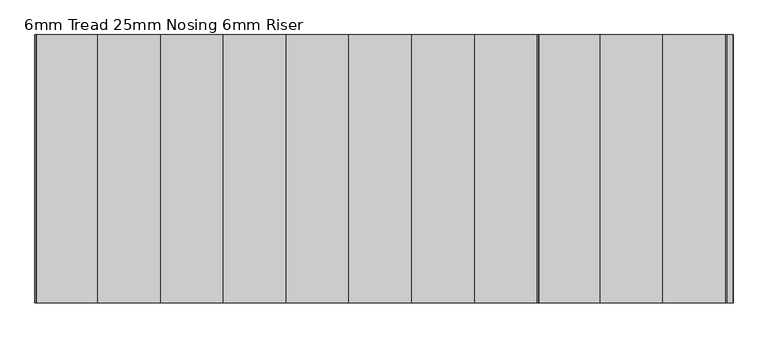
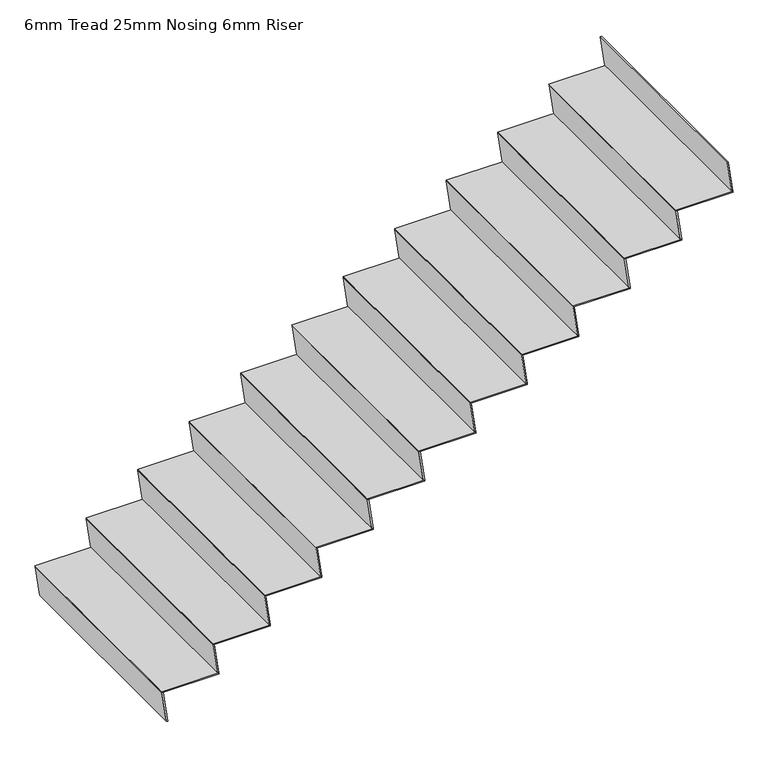
"""IFC4 building model written with IfcOpenShell, lengths in millimetres: stair flight geometry, 6mm Tread 25mm Nosing 6mm Riser."""

import ifcopenshell
import ifcopenshell.guid

model = None  # the IFC model being written
_history = None  # IfcOwnerHistory: only IFC2X3 demands one
_inside = {}  # id of a spatial element -> (the spatial element, [elements in it])
_under = {}  # id of a project, library or spatial element -> (it, [spatial elements below it])
_declared = {}  # id of a project -> (the project, [libraries it declares])
_typed = {}  # id of a type object -> (the type object, [elements of that type])
_made_of = {}  # id of a material, layer set ... -> (it, [elements and type objects made of it])


def new_model(schema):
    """Start an empty IFC model of exactly this schema.

    Asked for "IFC4X3", IfcOpenShell would pick the latest addendum, in which some entities
    have other attributes; the version numbers below select the first issue.
    IFC2X3 requires an IfcOwnerHistory on every rooted entity: one is made here for all.
    """
    global model, _history
    if schema == "IFC4X3":
        model = ifcopenshell.file(schema_version=(4, 3, 0, 0))
    else:
        model = ifcopenshell.file(schema=schema)
    _inside.clear()
    _under.clear()
    _declared.clear()
    _typed.clear()
    _made_of.clear()
    _history = None
    if model.schema == "IFC2X3":
        org = make("IfcOrganization", Name="unknown")
        user = make(
            "IfcPersonAndOrganization",
            ThePerson=make("IfcPerson", FamilyName="unknown"),
            TheOrganization=org,
        )
        app = make(
            "IfcApplication",
            ApplicationDeveloper=org,
            Version="unknown",
            ApplicationFullName="unknown",
            ApplicationIdentifier="unknown",
        )
        _history = make(
            "IfcOwnerHistory",
            OwningUser=user,
            OwningApplication=app,
            ChangeAction="ADDED",
            CreationDate=0,
        )
    return model


def make(cls, **values):
    """One entity of the class cls with the attributes given. An attribute that is None is left unset."""
    return model.create_entity(
        cls, **{name: value for name, value in values.items() if value is not None}
    )


def rooted(cls, **values):
    """An entity with a GlobalId (a new one), such as an element, a storey or a relation."""
    return make(cls, GlobalId=ifcopenshell.guid.new(), OwnerHistory=_history, **values)


def si_unit(unit_type, name, prefix=None):
    """IfcSIUnit, for example si_unit("LENGTHUNIT", "METRE", prefix="MILLI")."""
    return make("IfcSIUnit", UnitType=unit_type, Prefix=prefix, Name=name)


def assignment(units):
    """IfcUnitAssignment: the units of a project."""
    return None if units is None else make("IfcUnitAssignment", Units=units)


def point(xyz):
    """IfcCartesianPoint."""
    return None if xyz is None else make("IfcCartesianPoint", Coordinates=xyz)


def direction(xyz):
    """IfcDirection."""
    return None if xyz is None else make("IfcDirection", DirectionRatios=xyz)


def frame(location, z_axis=None, x_axis=None):
    """IfcAxis2Placement3D, a coordinate frame: its origin and axes. An axis left out is left unset."""
    return make(
        "IfcAxis2Placement3D",
        Location=point(location),
        Axis=direction(z_axis),
        RefDirection=direction(x_axis),
    )


def origin():
    """The frame at (0, 0, 0) with its axes left unset."""
    return frame((0.0, 0.0, 0.0))


def place(relative_to, where):
    """IfcLocalPlacement: puts the frame where relative to a parent placement (None: the world)."""
    return make(
        "IfcLocalPlacement", PlacementRelTo=relative_to, RelativePlacement=where
    )


def context(
    kind, dimensions, precision=None, world=None, true_north=None, identifier=None
):
    """IfcGeometricRepresentationContext, for example the 3D "Model" context."""
    return make(
        "IfcGeometricRepresentationContext",
        ContextIdentifier=identifier,
        ContextType=kind,
        CoordinateSpaceDimension=dimensions,
        Precision=precision,
        WorldCoordinateSystem=world,
        TrueNorth=true_north,
    )


def project(units=None, contexts=None):
    """IfcProject with its units and contexts."""
    return rooted(
        "IfcProject",
        Name="project",
        RepresentationContexts=contexts,
        UnitsInContext=assignment(units),
    )


def spatial(cls, under=None, at=None, **own):
    """A site, building, storey or space (cls), placed at a placement, below another one or the project."""
    s = rooted(cls, ObjectPlacement=at, **own)
    if under is not None:
        _under.setdefault(under.id(), (under, []))[1].append(s)
    return s


def polyline(points):
    """IfcPolyline through the points."""
    return make("IfcPolyline", Points=[point(p) for p in points])


def outline(outer, holes=None, kind="AREA"):
    """IfcArbitraryClosedProfileDef: a profile drawn as a closed curve; with holes, ...WithVoids."""
    if holes is None:
        return make("IfcArbitraryClosedProfileDef", ProfileType=kind, OuterCurve=outer)
    return make(
        "IfcArbitraryProfileDefWithVoids",
        ProfileType=kind,
        OuterCurve=outer,
        InnerCurves=holes,
    )


def extrude(swept, where, along, depth):
    """IfcExtrudedAreaSolid: the profile swept, set in the frame where, extruded along a direction by depth."""
    return make(
        "IfcExtrudedAreaSolid",
        SweptArea=swept,
        Position=where,
        ExtrudedDirection=direction(along),
        Depth=depth,
    )


def shape(context_of_items, identifier, shape_type, items):
    """IfcShapeRepresentation: the items that make up one representation, for example the "Body"."""
    return make(
        "IfcShapeRepresentation",
        ContextOfItems=context_of_items,
        RepresentationIdentifier=identifier,
        RepresentationType=shape_type,
        Items=items,
    )


def source(mapping_origin, context_of_items, identifier, shape_type, items):
    """IfcRepresentationMap: a shape defined once, which mapped items show again and again."""
    return make(
        "IfcRepresentationMap",
        MappingOrigin=mapping_origin,
        MappedRepresentation=shape(context_of_items, identifier, shape_type, items),
    )


def transform(
    local_origin,
    x_axis=None,
    y_axis=None,
    z_axis=None,
    scale=None,
    scale2=None,
    scale3=None,
    uniform=True,
):
    """IfcCartesianTransformationOperator3D, or its non-uniform kind. x_axis, y_axis, z_axis: its Axis1, 2, 3."""
    if uniform:
        return make(
            "IfcCartesianTransformationOperator3D",
            Axis1=direction(x_axis),
            Axis2=direction(y_axis),
            LocalOrigin=point(local_origin),
            Scale=scale,
            Axis3=direction(z_axis),
        )
    return make(
        "IfcCartesianTransformationOperator3DnonUniform",
        Axis1=direction(x_axis),
        Axis2=direction(y_axis),
        LocalOrigin=point(local_origin),
        Scale=scale,
        Axis3=direction(z_axis),
        Scale2=scale2,
        Scale3=scale3,
    )


def mapped(mapping_source, mapping_target):
    """IfcMappedItem: shows the shape of a source again, moved by a transform."""
    return make(
        "IfcMappedItem", MappingSource=mapping_source, MappingTarget=mapping_target
    )


def made_of(thing, what):
    """Note that an element or type object is made of a material, layer set ...; save() writes the relation."""
    if what is not None:
        _made_of.setdefault(what.id(), (what, []))[1].append(thing)
    return thing


def element(
    cls,
    number,
    at=None,
    inside=None,
    cuts=None,
    type_object=None,
    material=None,
    context=None,
    identifier="Body",
    shape_type=None,
    held_by="IfcProductDefinitionShape",
    body=None,
    shapes=None,
    **own,
):
    """One element of the class cls, such as IfcWall. Its Tag is "e" and its number.

    at: its placement. inside: the storey or other place that contains it. cuts: it is an
    opening in that element (IfcRelVoidsElement). A single representation is given by context,
    identifier, shape_type and body (its items); several are given by shapes. held_by: the class
    of the entity that holds the representations. save() writes the other relations.
    """
    e = rooted(cls, Tag="e%d" % number, ObjectPlacement=at, **own)
    if body is not None:
        shapes = [shape(context, identifier, shape_type, body)]
    if shapes is not None:
        e.Representation = make(held_by, Representations=shapes)
    if inside is not None:
        _inside.setdefault(inside.id(), (inside, []))[1].append(e)
    if cuts is not None:
        rooted(
            "IfcRelVoidsElement", RelatingBuildingElement=cuts, RelatedOpeningElement=e
        )
    if type_object is not None:
        _typed.setdefault(type_object.id(), (type_object, []))[1].append(e)
    return made_of(e, material)


def aggregate(whole, parts):
    """IfcRelAggregates: a whole, such as a stair, and the parts it consists of."""
    return rooted("IfcRelAggregates", RelatingObject=whole, RelatedObjects=parts)


def save(model, path):
    """Write the relations noted so far, then the file.

    IfcRelAggregates (storeys below a building ...), IfcRelContainedInSpatialStructure (elements
    in a storey), IfcRelDefinesByType, IfcRelAssociatesMaterial and IfcRelDeclares: one each for
    every whole, place, type object, material and project.
    """
    for whole, parts in _under.values():
        aggregate(whole, parts)
    for where, things in _inside.values():
        rooted(
            "IfcRelContainedInSpatialStructure",
            RelatedElements=things,
            RelatingStructure=where,
        )
    for kind, things in _typed.values():
        rooted("IfcRelDefinesByType", RelatedObjects=things, RelatingType=kind)
    for what, things in _made_of.values():
        rooted("IfcRelAssociatesMaterial", RelatedObjects=things, RelatingMaterial=what)
    for by, libraries in _declared.values():
        rooted("IfcRelDeclares", RelatingContext=by, RelatedDefinitions=libraries)
    model.write(path)


def stair_flight_6mm_tread_25mm_nosing_6mm_riser_ed312722(model_context):
    return source(origin(), model_context, "Body", "SweptSolid", [
        extrude(outline(polyline([(28647.0588235, 13631.0599092), (28647.0588235, 13325.0), (28641.0588235, 13325.85), (28641.0588235, 13631.9099092), (28647.0588235, 13631.0599092)])), frame((0.0, 10220.4345331, 0.0), z_axis=(0.0, 1.0, 0.0), x_axis=(0.0, 0.0, 1.0)), (0.0, 0.0, 1.0), 1175.0),
        extrude(outline(polyline([(28641.0588235, 13325.85), (28470.5882353, 13350.0), (28470.5882353, 13356.0599092), (28641.0588235, 13331.9099092), (28641.0588235, 13325.85)])), frame((0.0, 10220.4345331, 0.0), z_axis=(0.0, 1.0, 0.0), x_axis=(0.0, 0.0, 1.0)), (0.0, 0.0, 1.0), 1175.0),
        extrude(outline(polyline([(28817.5294118, 13600.85), (28647.0588235, 13625.0), (28647.0588235, 13631.0599092), (28817.5294118, 13606.9099092), (28817.5294118, 13600.85)])), frame((0.0, 10220.4345331, 0.0), z_axis=(0.0, 1.0, 0.0), x_axis=(0.0, 0.0, 1.0)), (0.0, 0.0, 1.0), 1175.0),
        extrude(outline(polyline([(28823.5294118, 13906.0599092), (28823.5294118, 13600.0), (28817.5294118, 13600.85), (28817.5294118, 13906.9099092), (28823.5294118, 13906.0599092)])), frame((0.0, 10220.4345331, 0.0), z_axis=(0.0, 1.0, 0.0), x_axis=(0.0, 0.0, 1.0)), (0.0, 0.0, 1.0), 1175.0),
        extrude(outline(polyline([(28994.0, 13875.85), (28823.5294118, 13900.0), (28823.5294118, 13906.0599092), (28994.0, 13881.9099092), (28994.0, 13875.85)])), frame((0.0, 10220.4345331, 0.0), z_axis=(0.0, 1.0, 0.0), x_axis=(0.0, 0.0, 1.0)), (0.0, 0.0, 1.0), 1175.0),
        extrude(outline(polyline([(29000.0, 14181.0599092), (29000.0, 13875.0), (28994.0, 13875.85), (28994.0, 14181.9099092), (29000.0, 14181.0599092)])), frame((0.0, 10220.4345331, 0.0), z_axis=(0.0, 1.0, 0.0), x_axis=(0.0, 0.0, 1.0)), (0.0, 0.0, 1.0), 1175.0),
        extrude(outline(polyline([(29170.4705882, 14150.85), (29000.0, 14175.0), (29000.0, 14181.0599092), (29170.4705882, 14156.9099092), (29170.4705882, 14150.85)])), frame((0.0, 10220.4345331, 0.0), z_axis=(0.0, 1.0, 0.0), x_axis=(0.0, 0.0, 1.0)), (0.0, 0.0, 1.0), 1175.0),
        extrude(outline(polyline([(29176.4705882, 14456.0599092), (29176.4705882, 14150.0), (29170.4705882, 14150.85), (29170.4705882, 14456.9099092), (29176.4705882, 14456.0599092)])), frame((0.0, 10220.4345331, 0.0), z_axis=(0.0, 1.0, 0.0), x_axis=(0.0, 0.0, 1.0)), (0.0, 0.0, 1.0), 1175.0),
        extrude(outline(polyline([(29346.9411765, 14425.85), (29176.4705882, 14450.0), (29176.4705882, 14456.0599092), (29346.9411765, 14431.9099092), (29346.9411765, 14425.85)])), frame((0.0, 10220.4345331, 0.0), z_axis=(0.0, 1.0, 0.0), x_axis=(0.0, 0.0, 1.0)), (0.0, 0.0, 1.0), 1175.0),
        extrude(outline(polyline([(29352.9411765, 14731.0599092), (29352.9411765, 14425.0), (29346.9411765, 14425.85), (29346.9411765, 14731.9099092), (29352.9411765, 14731.0599092)])), frame((0.0, 10220.4345331, 0.0), z_axis=(0.0, 1.0, 0.0), x_axis=(0.0, 0.0, 1.0)), (0.0, 0.0, 1.0), 1175.0),
        extrude(outline(polyline([(29523.4117647, 14700.85), (29352.9411765, 14725.0), (29352.9411765, 14731.0599092), (29523.4117647, 14706.9099092), (29523.4117647, 14700.85)])), frame((0.0, 10220.4345331, 0.0), z_axis=(0.0, 1.0, 0.0), x_axis=(0.0, 0.0, 1.0)), (0.0, 0.0, 1.0), 1175.0),
        extrude(outline(polyline([(29529.4117647, 15006.0599092), (29529.4117647, 14700.0), (29523.4117647, 14700.85), (29523.4117647, 15006.9099092), (29529.4117647, 15006.0599092)])), frame((0.0, 10220.4345331, 0.0), z_axis=(0.0, 1.0, 0.0), x_axis=(0.0, 0.0, 1.0)), (0.0, 0.0, 1.0), 1175.0),
        extrude(outline(polyline([(29699.8823529, 14975.85), (29529.4117647, 15000.0), (29529.4117647, 15006.0599092), (29699.8823529, 14981.9099092), (29699.8823529, 14975.85)])), frame((0.0, 10220.4345331, 0.0), z_axis=(0.0, 1.0, 0.0), x_axis=(0.0, 0.0, 1.0)), (0.0, 0.0, 1.0), 1175.0),
        extrude(outline(polyline([(29705.8823529, 15281.0599092), (29705.8823529, 14975.0), (29699.8823529, 14975.85), (29699.8823529, 15281.9099092), (29705.8823529, 15281.0599092)])), frame((0.0, 10220.4345331, 0.0), z_axis=(0.0, 1.0, 0.0), x_axis=(0.0, 0.0, 1.0)), (0.0, 0.0, 1.0), 1175.0),
        extrude(outline(polyline([(29876.3529412, 15250.85), (29705.8823529, 15275.0), (29705.8823529, 15281.0599092), (29876.3529412, 15256.9099092), (29876.3529412, 15250.85)])), frame((0.0, 10220.4345331, 0.0), z_axis=(0.0, 1.0, 0.0), x_axis=(0.0, 0.0, 1.0)), (0.0, 0.0, 1.0), 1175.0),
        extrude(outline(polyline([(29882.3529412, 15556.0599092), (29882.3529412, 15250.0), (29876.3529412, 15250.85), (29876.3529412, 15556.9099092), (29882.3529412, 15556.0599092)])), frame((0.0, 10220.4345331, 0.0), z_axis=(0.0, 1.0, 0.0), x_axis=(0.0, 0.0, 1.0)), (0.0, 0.0, 1.0), 1175.0),
        extrude(outline(polyline([(30052.8235294, 15525.85), (29882.3529412, 15550.0), (29882.3529412, 15556.0599092), (30052.8235294, 15531.9099092), (30052.8235294, 15525.85)])), frame((0.0, 10220.4345331, 0.0), z_axis=(0.0, 1.0, 0.0), x_axis=(0.0, 0.0, 1.0)), (0.0, 0.0, 1.0), 1175.0),
        extrude(outline(polyline([(30058.8235294, 15831.0599092), (30058.8235294, 15525.0), (30052.8235294, 15525.85), (30052.8235294, 15831.9099092), (30058.8235294, 15831.0599092)])), frame((0.0, 10220.4345331, 0.0), z_axis=(0.0, 1.0, 0.0), x_axis=(0.0, 0.0, 1.0)), (0.0, 0.0, 1.0), 1175.0),
        extrude(outline(polyline([(30229.2941176, 15800.85), (30058.8235294, 15825.0), (30058.8235294, 15831.0599092), (30229.2941176, 15806.9099092), (30229.2941176, 15800.85)])), frame((0.0, 10220.4345331, 0.0), z_axis=(0.0, 1.0, 0.0), x_axis=(0.0, 0.0, 1.0)), (0.0, 0.0, 1.0), 1175.0),
        extrude(outline(polyline([(30235.2941176, 16106.0599092), (30235.2941176, 15800.0), (30229.2941176, 15800.85), (30229.2941176, 16106.9099092), (30235.2941176, 16106.0599092)])), frame((0.0, 10220.4345331, 0.0), z_axis=(0.0, 1.0, 0.0), x_axis=(0.0, 0.0, 1.0)), (0.0, 0.0, 1.0), 1175.0),
        extrude(outline(polyline([(30405.7647059, 16075.85), (30235.2941176, 16100.0), (30235.2941176, 16106.0599092), (30405.7647059, 16081.9099092), (30405.7647059, 16075.85)])), frame((0.0, 10220.4345331, 0.0), z_axis=(0.0, 1.0, 0.0), x_axis=(0.0, 0.0, 1.0)), (0.0, 0.0, 1.0), 1175.0),
        extrude(outline(polyline([(30582.2352941, 16350.85), (30411.7647059, 16375.0), (30411.7647059, 16381.0599092), (30582.2352941, 16356.9099092), (30582.2352941, 16350.85)])), frame((0.0, 10220.4345331, 0.0), z_axis=(0.0, 1.0, 0.0), x_axis=(0.0, 0.0, 1.0)), (0.0, 0.0, 1.0), 1175.0),
        extrude(outline(polyline([(30411.7647059, 16381.0599092), (30411.7647059, 16075.0), (30405.7647059, 16075.85), (30405.7647059, 16381.9099092), (30411.7647059, 16381.0599092)])), frame((0.0, 10220.4345331, 0.0), z_axis=(0.0, 1.0, 0.0), x_axis=(0.0, 0.0, 1.0)), (0.0, 0.0, 1.0), 1175.0),
    ])


if __name__ == "__main__":
    model = new_model("IFC4")
    model_context = context("Model", 3, world=origin())
    ifc_project = project(units=[si_unit("LENGTHUNIT", "METRE", prefix="MILLI")], contexts=[model_context])
    site = spatial("IfcSite", under=ifc_project)
    building = spatial("IfcBuilding", under=site)
    placement = place(None, origin())
    stair_flight_6mm_tread_25mm_nosing_6mm_riser_shape = stair_flight_6mm_tread_25mm_nosing_6mm_riser_ed312722(model_context)
    element("IfcStairFlight", 1, ObjectType="6mm Tread 25mm Nosing 6mm Riser", at=placement, inside=building, context=model_context, shape_type="MappedRepresentation", body=[
        mapped(stair_flight_6mm_tread_25mm_nosing_6mm_riser_shape, transform((0.0, 0.0, 0.0), x_axis=(1.0, 0.0, 0.0), y_axis=(0.0, 1.0, 0.0), z_axis=(0.0, 0.0, 1.0))),
    ])
    save(model, "model.ifc")

# Revit data of these elements
# Element 1 (IfcStairFlight, "6mm Tread 25mm Nosing 6mm Riser")
#   Materials on its faces: "Steel, Paint Finish, Dark Gray"
# Materials
#   "Steel, Paint Finish, Dark Gray": class "Metal", colour RGB 89 89 89, transparency 0, Description = "Steel, paint finish, dark gray, glossy", Cost = 0
